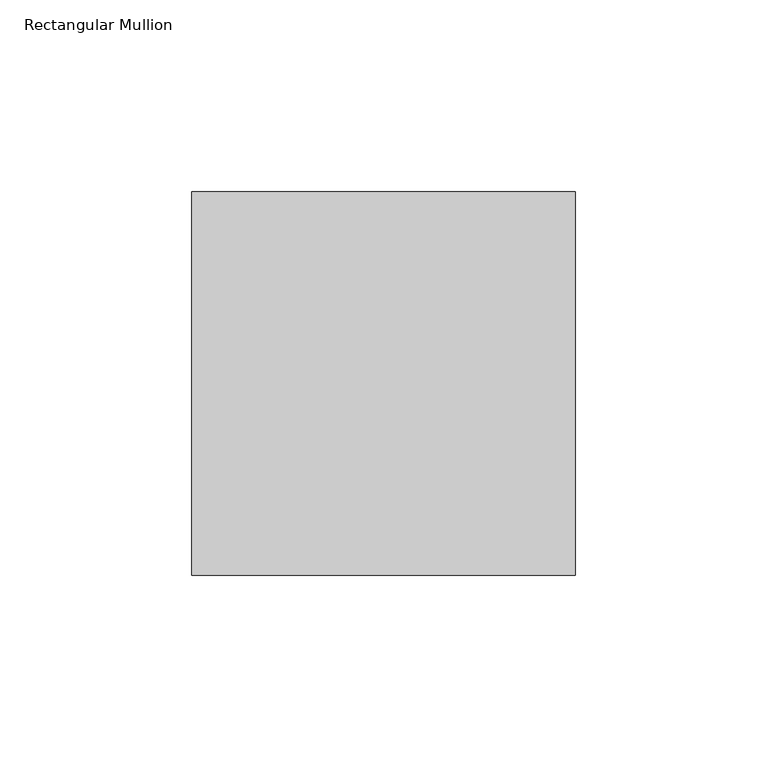
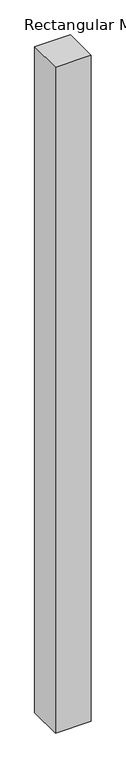
"""IFC4 building model written with IfcOpenShell, lengths in millimetres: member geometry, Rectangular Mullion : 알루미늄_Rectangular Cap_100 x100."""

from ifc_helpers import new_model, si_unit, frame, origin, place, context, project, spatial, polyline, outline, extrude, source, transform, mapped, element, save


def rectangular_mullion_4956deae(model_context):
    return source(origin(), model_context, "Body", "SweptSolid", [
        extrude(outline(polyline([(0.0, 50.0), (0.0, -50.0), (-100.0, -50.0), (-100.0, 50.0), (0.0, 50.0)])), frame((0.0, 0.0, -1961.9999999), z_axis=(0.0, 0.0, 1.0), x_axis=(1.0, 0.0, 0.0)), (0.0, 0.0, 1.0), 1961.9999999),
    ])


if __name__ == "__main__":
    model = new_model("IFC4")
    model_context = context("Model", 3, world=origin())
    ifc_project = project(units=[si_unit("LENGTHUNIT", "METRE", prefix="MILLI")], contexts=[model_context])
    site = spatial("IfcSite", under=ifc_project)
    building = spatial("IfcBuilding", under=site)
    placement = place(None, origin())
    rectangular_mullion_shape = rectangular_mullion_4956deae(model_context)
    element("IfcMember", 1, ObjectType="Rectangular Mullion : 알루미늄_Rectangular Cap_100 x100", at=placement, inside=building, context=model_context, shape_type="MappedRepresentation", body=[
        mapped(rectangular_mullion_shape, transform((0.0, 0.0, 0.0), x_axis=(1.0, 0.0, 0.0), y_axis=(0.0, 1.0, 0.0), z_axis=(0.0, 0.0, 1.0))),
    ])
    save(model, "model.ifc")

# Revit data of these elements
# Type "Rectangular Mullion : 알루미늄_Rectangular Cap_100 x100"
#   built-in parameter 1007304 = 0.328084 (stored number, unit not read)
#   built-in parameter 1007301 = 0.164042 (stored number, unit not read)
#   built-in parameter 1007300 = 0.164042 (stored number, unit not read)
# Element 1 (IfcMember, "Rectangular Mullion : 알루미늄_Rectangular Cap_100 x100")
#   Materials on its faces: "00_Metal_Stainless Steel"
# Materials
#   "00_Metal_Stainless Steel": class "Metal", colour RGB 148 148 148, transparency 0, Description = "Steel", Cost = 0
